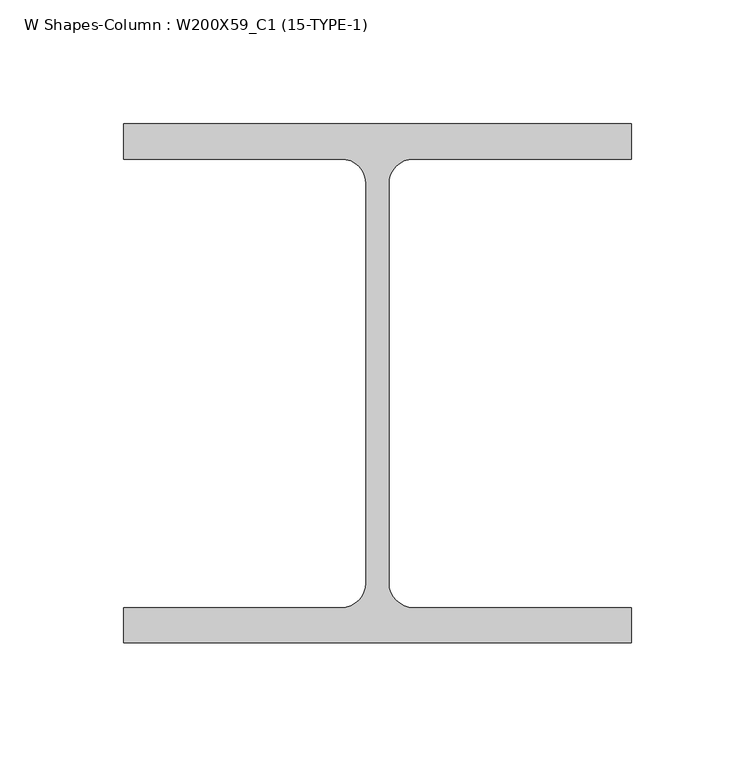
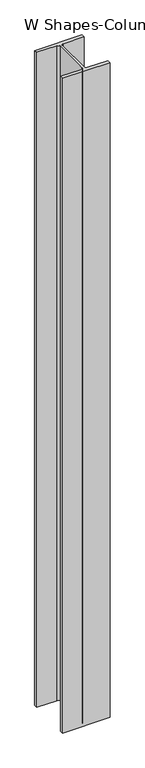
"""IFC4 building model written with IfcOpenShell, lengths in millimetres: column geometry, W Shapes-Column : W200X59_C1 (15-TYPE-1)."""

from ifc_helpers import new_model, si_unit, point, frame, frame_2d, origin, place, context, project, spatial, polyline, circle_curve, trimmed, segment, composite_curve, outline, extrude, source, transform, mapped, element, save


def w_shapes_column_w200x59_c1_15_type_1_032f0c05(model_context):
    return source(origin(), model_context, "Body", "SweptSolid", [
        extrude(outline(composite_curve([segment(polyline([(102.489, 104.775), (102.489, 90.551), (14.5796, 90.551)]), True, "CONTINUOUS"), segment(trimmed(circle_curve(frame_2d((14.5796, 80.5434)), 10.0076), [point((14.5796, 90.551))], [point((4.572, 80.5434))], True, "CARTESIAN"), True, "CONTINUOUS"), segment(polyline([(4.572, 80.5434), (4.572, -80.5434)]), True, "CONTINUOUS"), segment(trimmed(circle_curve(frame_2d((14.5796, -80.5434)), 10.0076), [point((4.572, -80.5434))], [point((14.5796, -90.551))], True, "CARTESIAN"), True, "CONTINUOUS"), segment(polyline([(14.5796, -90.551), (102.489, -90.551), (102.489, -104.775), (-102.489, -104.775), (-102.489, -90.551), (-14.5796, -90.551)]), True, "CONTINUOUS"), segment(trimmed(circle_curve(frame_2d((-14.5796, -80.5434)), 10.0076), [point((-14.5796, -90.551))], [point((-4.572, -80.5434))], True, "CARTESIAN"), True, "CONTINUOUS"), segment(polyline([(-4.572, -80.5434), (-4.572, 80.5434)]), True, "CONTINUOUS"), segment(trimmed(circle_curve(frame_2d((-14.5796, 80.5434)), 10.0076), [point((-4.572, 80.5434))], [point((-14.5796, 90.551))], True, "CARTESIAN"), True, "CONTINUOUS"), segment(polyline([(-14.5796, 90.551), (-102.489, 90.551), (-102.489, 104.775), (102.489, 104.775)]), True, "CONTINUOUS")], self_intersect=False)), frame((0.0, 0.0, 6240.0), z_axis=(0.0, 0.0, 1.0), x_axis=(1.0, 0.0, 0.0)), (0.0, 0.0, 1.0), 3000.0),
    ])


if __name__ == "__main__":
    model = new_model("IFC4")
    model_context = context("Model", 3, world=origin())
    ifc_project = project(units=[si_unit("LENGTHUNIT", "METRE", prefix="MILLI")], contexts=[model_context])
    site = spatial("IfcSite", under=ifc_project)
    building = spatial("IfcBuilding", under=site)
    placement = place(None, origin())
    w_shapes_column_w200x59_c1_15_type_1_shape = w_shapes_column_w200x59_c1_15_type_1_032f0c05(model_context)
    element("IfcColumn", 1, ObjectType="W Shapes-Column : W200X59_C1 (15-TYPE-1)", at=placement, inside=building, context=model_context, shape_type="MappedRepresentation", body=[
        mapped(w_shapes_column_w200x59_c1_15_type_1_shape, transform((0.0, 0.0, 0.0), x_axis=(1.0, 0.0, 0.0), y_axis=(0.0, 1.0, 0.0), z_axis=(0.0, 0.0, 1.0))),
    ])
    save(model, "model.ifc")

# Revit data of these elements
# Type "W Shapes-Column : W200X59_C1 (15-TYPE-1)"
#   Section Name Key = "W8x40"
#   Assembly Code = "B10"
#   Width = 20.4978 cm
#   Web Thickness = 0.9144 cm
#   Web Fillet = 1.0008 cm
#   Warping Constant = 194957.0 cm⁶
#   Torsional Moment of Inertia = 46.6179 cm⁴
#   Section Area = 75.4837 cm²
#   Plastic Modulus weak axis = 303.161 cm³
#   Plastic Modulus strong axis = 652.205 cm³
#   Perimeter = 1.20396 m²/m
#   Nominal Weight = 59.5266 kgf/m
#   Moment of Inertia weak axis = 2043.70 cm⁴
#   Moment of Inertia strong axis = 6076.98 cm⁴
#   Height = 20.955 cm
#   Flange Thickness = 1.4224 cm
#   Elastic Modulus weak axis = 199.922 cm³
#   Elastic Modulus strong axis = 581.741 cm³
#   Clear Web Height = 19.05 cm
#   Centroid Vertical = 10.4775 cm
#   Centroid Horizontal = 10.2489 cm
#   Bolt Spacing = 13.97 cm
#   Structural Material [instance default] = Steel ASTM A992
#   Principal Axes Angle = 0
# Element 1 (IfcColumn, "W Shapes-Column : W200X59_C1 (15-TYPE-1)")
#   Structural Material = none
# Materials
#   "Steel ASTM A992": class "Metal", colour RGB 199 199 199, transparency 0, Description = "Structural steel 50ksi", Cost = 0
